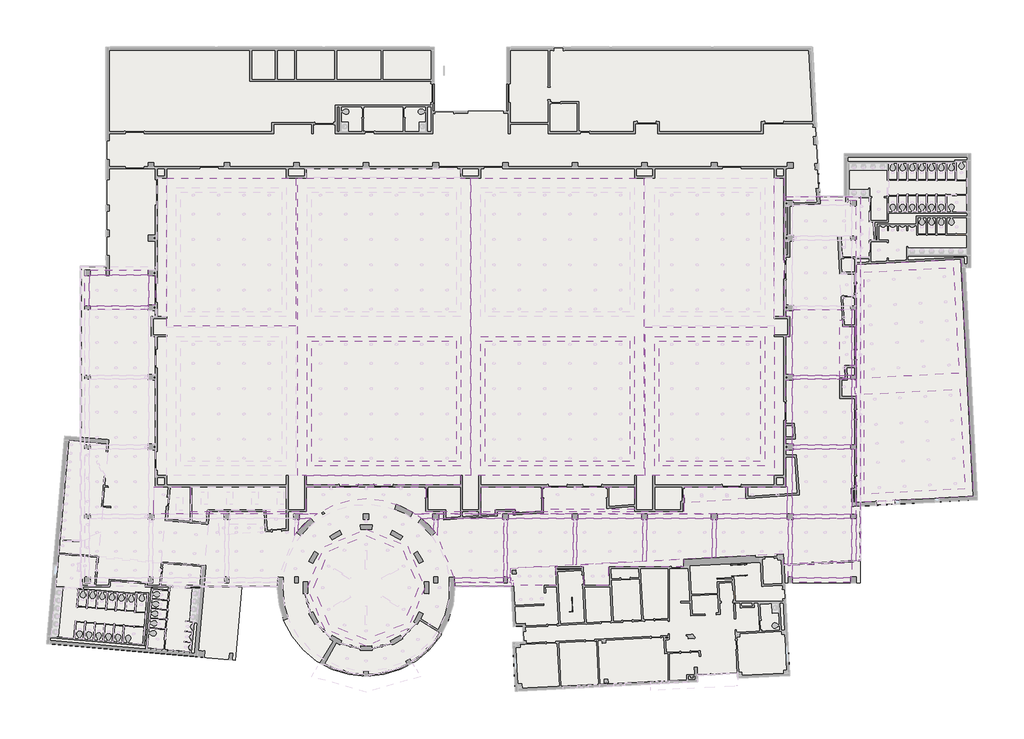
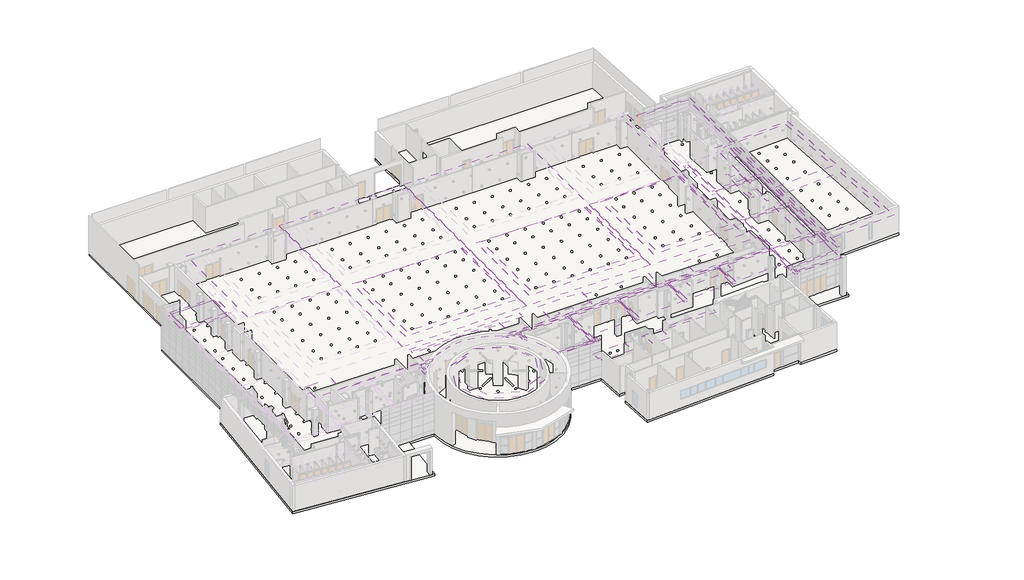
# One storey, part 23 of 30: 71 coverings, 1 slab.
"""IFC4 building model written with IfcOpenShell, lengths in millimetres."""

from ifc_helpers import new_model, si_unit, point, frame, frame_2d, origin, place, context, project, spatial, polyline, circle_curve, trimmed, segment, composite_curve, outline, extrude, faceted_brep, element, save

model = new_model("IFC4")

# Units and contexts
model_context = context("Model", 3, world=origin())
ifc_project = project(units=[si_unit("LENGTHUNIT", "METRE", prefix="MILLI")], contexts=[model_context])

# Site, building, storey
site = spatial("IfcSite", under=ifc_project)
building = spatial("IfcBuilding", under=site)
storey = spatial("IfcBuildingStorey", under=building, Name="1ST. FL.", Elevation=0.0)

# Coverings
placement = place(None, origin())
element("IfcCovering", 1, ObjectType="2' x 2' ACT System", at=placement, inside=storey, context=model_context, shape_type="SweptSolid", body=[
    extrude(outline(polyline([(-29897.3440345, -14000.959635), (-29897.3440345, -2418.559635), (-15978.1440345, -2418.559635), (-15978.1440345, -14000.959635), (-29897.3440345, -14000.959635)])), frame((0.0, 0.0, 6096.0), z_axis=(0.0, 0.0, 1.0), x_axis=(1.0, 0.0, 0.0)), (0.0, 0.0, 1.0), 50.8),
])
element("IfcCovering", 2, ObjectType="2' x 2' ACT System", at=placement, inside=storey, context=model_context, shape_type="SweptSolid", body=[
    extrude(outline(polyline([(13333.4559655, -14000.959635), (3579.8559655, -14000.959635), (3579.8559655, -2418.559635), (13333.4559655, -2418.559635), (13333.4559655, -14000.959635)])), frame((0.0, 0.0, 6096.0), z_axis=(0.0, 0.0, 1.0), x_axis=(1.0, 0.0, 0.0)), (0.0, 0.0, 1.0), 50.8),
])
element("IfcCovering", 3, ObjectType="2' x 2' ACT System", at=placement, inside=storey, context=model_context, shape_type="SweptSolid", body=[
    extrude(outline(polyline([(735.0559655, -14000.959635), (-13184.1440345, -14000.959635), (-13184.1440345, -2418.559635), (735.0559655, -2418.559635), (735.0559655, -14000.959635)])), frame((0.0, 0.0, 6096.0), z_axis=(0.0, 0.0, 1.0), x_axis=(1.0, 0.0, 0.0)), (0.0, 0.0, 1.0), 50.8),
])
element("IfcCovering", 4, ObjectType="2' x 2' ACT System", at=placement, inside=storey, context=model_context, shape_type="SweptSolid", body=[
    extrude(outline(polyline([(16476.7059655, -5717.384635), (16476.7059655, -5625.309635), (16384.6309655, -5625.309635), (16384.6309655, 534.190365), (16476.7059655, 534.190365), (16476.7059655, 626.265365), (22118.6809655, 626.265365), (22118.6809655, -5717.384635), (16476.7059655, -5717.384635)])), frame((0.0, 0.0, 5181.6), z_axis=(0.0, 0.0, 1.0), x_axis=(1.0, 0.0, 0.0)), (0.0, 0.0, 1.0), 50.8),
])
element("IfcCovering", 5, ObjectType="2' x 2' ACT System", at=placement, inside=storey, context=model_context, shape_type="SweptSolid", body=[
    extrude(outline(polyline([(16476.7059655, -6079.334635), (22118.6809655, -6079.334635), (22118.6809655, -12422.984635), (16476.7059655, -12422.984635), (16476.7059655, -12330.909635), (16384.6309655, -12330.909635), (16384.6309655, -6171.409635), (16476.7059655, -6171.409635), (16476.7059655, -6079.334635)])), frame((0.0, 0.0, 5181.6), z_axis=(0.0, 0.0, 1.0), x_axis=(1.0, 0.0, 0.0)), (0.0, 0.0, 1.0), 50.8),
])
element("IfcCovering", 6, ObjectType="2' x 2' ACT System", at=placement, inside=storey, context=model_context, shape_type="SweptSolid", body=[
    extrude(outline(polyline([(16476.7059655, -19128.584635), (16476.7059655, -19036.509635), (16384.6309655, -19036.509635), (16384.6309655, -12877.009635), (16476.7059655, -12877.009635), (16476.7059655, -12784.934635), (22118.6809655, -12784.934635), (22118.6809655, -19128.584635), (16476.7059655, -19128.584635)])), frame((0.0, 0.0, 5181.6), z_axis=(0.0, 0.0, 1.0), x_axis=(1.0, 0.0, 0.0)), (0.0, 0.0, 1.0), 50.8),
])
element("IfcCovering", 7, ObjectType="2' x 2' ACT System", at=placement, inside=storey, context=model_context, shape_type="SweptSolid", body=[
    extrude(outline(polyline([(16476.7059655, -19490.534635), (22118.6809655, -19490.534635), (22118.6809655, -23584.9151815), (16384.6309655, -23885.4240083), (16384.6309655, -19582.609635), (16476.7059655, -19582.609635), (16476.7059655, -19490.534635)])), frame((0.0, 0.0, 5181.6), z_axis=(0.0, 0.0, 1.0), x_axis=(1.0, 0.0, 0.0)), (0.0, 0.0, 1.0), 50.8),
])
element("IfcCovering", 8, ObjectType="2' x 2' ACT System", at=placement, inside=storey, context=model_context, shape_type="SweptSolid", body=[
    extrude(outline(polyline([(15930.6059655, -19490.534635), (15930.6059655, -19582.609635), (16022.6809655, -19582.609635), (16022.6809655, -23904.393004), (15588.5919456, -23927.1426455), (15535.7509474, -22918.8763358), (9069.4309655, -23257.7618061), (9069.4309655, -19582.609635), (9161.5059655, -19582.609635), (9161.5059655, -19490.534635), (15930.6059655, -19490.534635)])), frame((0.0, 0.0, 5181.6), z_axis=(0.0, 0.0, 1.0), x_axis=(1.0, 0.0, 0.0)), (0.0, 0.0, 1.0), 50.8),
])
element("IfcCovering", 9, ObjectType="2' x 2' ACT System", at=placement, inside=storey, context=model_context, shape_type="SweptSolid", body=[
    extrude(outline(polyline([(2455.9059655, -19490.534635), (8615.4059655, -19490.534635), (8615.4059655, -19582.609635), (8707.4809655, -19582.609635), (8707.4809655, -23276.7308019), (2363.8309655, -23609.1874109), (2363.8309655, -19582.609635), (2455.9059655, -19582.609635), (2455.9059655, -19490.534635)])), frame((0.0, 0.0, 5181.6), z_axis=(0.0, 0.0, 1.0), x_axis=(1.0, 0.0, 0.0)), (0.0, 0.0, 1.0), 50.8),
])
element("IfcCovering", 10, ObjectType="2' x 2' ACT System", at=placement, inside=storey, context=model_context, shape_type="SweptSolid", body=[
    extrude(outline(polyline([(1909.8059655, -19490.534635), (1909.8059655, -19582.609635), (2001.8809655, -19582.609635), (2001.8809655, -23628.1564066), (-4341.7690345, -23960.6130157), (-4341.7690345, -19582.609635), (-4249.6940345, -19582.609635), (-4249.6940345, -19490.534635), (1909.8059655, -19490.534635)])), frame((0.0, 0.0, 5181.6), z_axis=(0.0, 0.0, 1.0), x_axis=(1.0, 0.0, 0.0)), (0.0, 0.0, 1.0), 50.8),
])
element("IfcCovering", 11, ObjectType="2' x 2' ACT System", at=placement, inside=storey, context=model_context, shape_type="SweptSolid", body=[
    extrude(outline(polyline([(-10955.2940345, -19490.534635), (-4795.7940345, -19490.534635), (-4795.7940345, -19582.609635), (-4703.7190345, -19582.609635), (-4703.7190345, -23979.5820114), (-10767.9512721, -24297.394956), (-10719.3593201, -25224.584635), (-11047.3690345, -25224.584635), (-11047.3690345, -19582.609635), (-10955.2940345, -19582.609635), (-10955.2940345, -19490.534635)])), frame((0.0, 0.0, 5181.6), z_axis=(0.0, 0.0, 1.0), x_axis=(1.0, 0.0, 0.0)), (0.0, 0.0, 1.0), 50.8),
])
element("IfcCovering", 12, ObjectType="2' x 2' ACT System", at=placement, inside=storey, context=model_context, shape_type="SweptSolid", body=[
    extrude(outline(polyline([(-45638.9940345, 3979.065365), (-45638.9940345, 3886.990365), (-45546.9190345, 3886.990365), (-45546.9190345, 1080.290365), (-45638.9940345, 1080.290365), (-45638.9940345, 988.215365), (-51280.9690345, 988.215365), (-51280.9690345, 3886.990365), (-51188.8940345, 3886.990365), (-51188.8940345, 3979.065365), (-45638.9940345, 3979.065365)])), frame((0.0, 0.0, 5181.6), z_axis=(0.0, 0.0, 1.0), x_axis=(1.0, 0.0, 0.0)), (0.0, 0.0, 1.0), 50.8),
])
element("IfcCovering", 13, ObjectType="2' x 2' ACT System", at=placement, inside=storey, context=model_context, shape_type="SweptSolid", body=[
    extrude(outline(composite_curve([segment(polyline([(-31072.0940345, -19490.534635), (-29954.9292989, -19490.534635)]), True, "CONTINUOUS"), segment(trimmed(circle_curve(frame_2d((-24639.5440345, -26167.559635)), 8534.4), [point((-29954.9292989, -19490.534635))], [point((-31164.1690345, -20666.1732671))], True, "CARTESIAN"), True, "CONTINUOUS"), segment(polyline([(-31164.1690345, -20666.1732671), (-31164.1690345, -19582.609635), (-31072.0940345, -19582.609635), (-31072.0940345, -19490.534635)]), True, "CONTINUOUS")], self_intersect=False)), frame((0.0, 0.0, 5181.6), z_axis=(0.0, 0.0, 1.0), x_axis=(1.0, 0.0, 0.0)), (0.0, 0.0, 1.0), 50.8),
])
element("IfcCovering", 14, ObjectType="2' x 2' ACT System", at=placement, inside=storey, context=model_context, shape_type="SweptSolid", body=[
    extrude(outline(composite_curve([segment(polyline([(-18206.9940345, -19490.534635), (-18206.9940345, -19582.609635), (-18114.9190345, -19582.609635), (-18114.9190345, -20666.1732671)]), True, "CONTINUOUS"), segment(trimmed(circle_curve(frame_2d((-24639.5440345, -26167.559635)), 8534.4), [point((-18114.9190345, -20666.1732671))], [point((-19324.1587701, -19490.534635))], True, "CARTESIAN"), True, "CONTINUOUS"), segment(polyline([(-19324.1587701, -19490.534635), (-18206.9940345, -19490.534635)]), True, "CONTINUOUS")], self_intersect=False)), frame((0.0, 0.0, 5181.6), z_axis=(0.0, 0.0, 1.0), x_axis=(1.0, 0.0, 0.0)), (0.0, 0.0, 1.0), 50.8),
])
element("IfcCovering", 15, ObjectType="2' x 2' ACT System", at=placement, inside=storey, context=model_context, shape_type="SweptSolid", body=[
    extrude(outline(composite_curve([segment(polyline([(-17660.8940345, -19490.534635), (-11501.3940345, -19490.534635), (-11501.3940345, -19582.609635), (-11409.3190345, -19582.609635), (-11409.3190345, -25224.584635), (-16157.3991696, -25224.584635)]), True, "CONTINUOUS"), segment(trimmed(circle_curve(frame_2d((-24639.5440345, -26167.559635)), 8534.4), [point((-16157.3991696, -25224.584635))], [point((-17752.9690345, -21126.620424))], True, "CARTESIAN"), True, "CONTINUOUS"), segment(polyline([(-17752.9690345, -21126.620424), (-17752.9690345, -19582.609635), (-17660.8940345, -19582.609635), (-17660.8940345, -19490.534635)]), True, "CONTINUOUS")], self_intersect=False)), frame((0.0, 0.0, 5181.6), z_axis=(0.0, 0.0, 1.0), x_axis=(1.0, 0.0, 0.0)), (0.0, 0.0, 1.0), 50.8),
])
element("IfcCovering", 16, ObjectType="2' x 2' ACT System", at=placement, inside=storey, context=model_context, shape_type="SweptSolid", body=[
    extrude(outline(polyline([(31909.2771996, 4687.1559255), (32443.7073352, -5510.3785431), (23334.7059655, -5987.7610764), (23334.7059655, 4237.7816888), (31909.2771996, 4687.1559255)])), frame((0.0, 0.0, 2743.2), z_axis=(0.0, 0.0, 1.0), x_axis=(1.0, 0.0, 0.0)), (0.0, 0.0, 1.0), 50.8),
])
element("IfcCovering", 17, ObjectType="2' x 2' ACT System", at=placement, inside=storey, context=model_context, shape_type="SweptSolid", body=[
    extrude(outline(polyline([(32523.4673326, -7032.2899541), (33027.0803286, -16641.7983694), (23334.7059655, -17149.7541858), (23334.7059655, -7513.8525317), (32523.4673326, -7032.2899541)])), frame((0.0, 0.0, 2743.2), z_axis=(0.0, 0.0, 1.0), x_axis=(1.0, 0.0, 0.0)), (0.0, 0.0, 1.0), 50.8),
])
element("IfcCovering", 18, ObjectType="GWB on Mtl. Stud", at=placement, inside=storey, context=model_context, shape_type="SweptSolid", body=[
    extrude(outline(polyline([(15594.0559655, -56.359635), (14679.6559655, -56.359635), (14679.6559655, 13304.040365), (15594.0559655, 13304.040365), (15594.0559655, -56.359635)])), frame((0.0, 0.0, 4572.0), z_axis=(0.0, 0.0, 1.0), x_axis=(1.0, 0.0, 0.0)), (0.0, 0.0, 1.0), 50.8),
    extrude(outline(polyline([(15594.0559655, -1986.759635), (15594.0559655, -15347.159635), (14679.6559655, -15347.159635), (14679.6559655, -1986.759635), (15594.0559655, -1986.759635)])), frame((0.0, 0.0, 4572.0), z_axis=(0.0, 0.0, 1.0), x_axis=(1.0, 0.0, 0.0)), (0.0, 0.0, 1.0), 50.8),
])
element("IfcCovering", 19, ObjectType="GWB on Mtl. Stud", at=placement, inside=storey, context=model_context, shape_type="Brep", body=[
    faceted_brep([(3148.0559655, -16261.559635, 4622.8), (14679.6559655, -16261.559635, 4622.8), (14679.6559655, -15397.959635, 4622.8), (14679.6559655, -15347.159635, 4622.8), (3148.0559655, -15347.159635, 4622.8), (3148.0559655, -15397.959635, 4622.8), (3148.0559655, -16261.559635, 4572.0), (3148.0559655, -15347.159635, 4572.0), (14679.6559655, -15347.159635, 4572.0), (14679.6559655, -16261.559635, 4572.0)], [[[0, 1, 2, 3, 4, 5]], [[6, 7, 8, 9]], [[1, 0, 6, 9]], [[3, 2, 1, 9, 8]], [[4, 3, 8, 7]], [[0, 5, 4, 7, 6]]]),
    faceted_brep([(-30379.9440345, -16261.559635, 4622.8), (-15546.3440345, -16261.559635, 4622.8), (-15546.3440345, -15397.959635, 4622.8), (-15546.3440345, -15347.159635, 4622.8), (-30379.9440345, -15347.159635, 4622.8), (-30379.9440345, -15397.959635, 4622.8), (-30379.9440345, -16261.559635, 4572.0), (-30379.9440345, -15347.159635, 4572.0), (-15546.3440345, -15347.159635, 4572.0), (-15546.3440345, -16261.559635, 4572.0)], [[[0, 1, 2, 3, 4, 5]], [[6, 7, 8, 9]], [[1, 0, 6, 9]], [[3, 2, 1, 9, 8]], [[4, 3, 8, 7]], [[0, 5, 4, 7, 6]]]),
    faceted_brep([(-43841.9440345, -16261.559635, 4622.8), (-32310.3440345, -16261.559635, 4622.8), (-32310.3440345, -15397.959635, 4622.8), (-32310.3440345, -15347.159635, 4622.8), (-43841.9440345, -15347.159635, 4622.8), (-43841.9440345, -15397.959635, 4622.8), (-43841.9440345, -16261.559635, 4572.0), (-43841.9440345, -15347.159635, 4572.0), (-32310.3440345, -15347.159635, 4572.0), (-32310.3440345, -16261.559635, 4572.0)], [[[0, 1, 2, 3, 4, 5]], [[6, 7, 8, 9]], [[1, 0, 6, 9]], [[3, 2, 1, 9, 8]], [[4, 3, 8, 7]], [[0, 5, 4, 7, 6]]]),
    faceted_brep([(1217.6559655, -16261.559635, 4622.8), (1217.6559655, -15397.959635, 4622.8), (1217.6559655, -15347.159635, 4622.8), (-13615.9440345, -15347.159635, 4622.8), (-13615.9440345, -15397.959635, 4622.8), (-13615.9440345, -16261.559635, 4622.8), (1217.6559655, -16261.559635, 4572.0), (-13615.9440345, -16261.559635, 4572.0), (-13615.9440345, -15347.159635, 4572.0), (1217.6559655, -15347.159635, 4572.0)], [[[0, 1, 2, 3, 4, 5]], [[6, 7, 8, 9]], [[2, 1, 0, 6, 9]], [[3, 2, 9, 8]], [[5, 4, 3, 8, 7]], [[0, 5, 7, 6]]]),
])
element("IfcCovering", 20, ObjectType="GWB on Mtl. Stud", at=placement, inside=storey, context=model_context, shape_type="SweptSolid", body=[
    extrude(outline(polyline([(-43841.9440345, 13304.040365), (-31395.9440345, 13304.040365), (-31395.9440345, -970.759635), (-43841.9440345, -970.759635), (-43841.9440345, 13304.040365)]), holes=[polyline([(-32310.3440345, -56.359635), (-32310.3440345, 12389.640365), (-42927.5440345, 12389.640365), (-42927.5440345, -56.359635), (-32310.3440345, -56.359635)])]), frame((0.0, 0.0, 5181.6), z_axis=(0.0, 0.0, 1.0), x_axis=(1.0, 0.0, 0.0)), (0.0, 0.0, 1.0), 50.8),
])
element("IfcCovering", 21, ObjectType="GWB on Mtl. Stud", at=placement, inside=storey, context=model_context, shape_type="Brep", body=[
    faceted_brep([(-31243.5440345, -15347.159635, 5232.4), (-30379.9440345, -15347.159635, 5232.4), (-15546.3440345, -15347.159635, 5232.4), (-14631.9440345, -15347.159635, 5232.4), (-14631.9440345, 13304.040365, 5232.4), (-15546.3440345, 13304.040365, 5232.4), (-30379.9440345, 13304.040365, 5232.4), (-31243.5440345, 13304.040365, 5232.4), (-15546.3440345, -14432.759635, 5232.4), (-30329.1440345, -14432.759635, 5232.4), (-30329.1440345, -1986.759635, 5232.4), (-15546.3440345, -1986.759635, 5232.4), (-15495.5440345, 12440.440365, 5232.4), (-15495.5440345, -107.159635, 5232.4), (-30379.9440345, -107.159635, 5232.4), (-30379.9440345, 12440.440365, 5232.4), (-14631.9440345, -15347.159635, 5181.6), (-31243.5440345, -15347.159635, 5181.6), (-31243.5440345, 13304.040365, 5181.6), (-14631.9440345, 13304.040365, 5181.6), (-30329.1440345, -14432.759635, 5181.6), (-15546.3440345, -14432.759635, 5181.6), (-15546.3440345, -1986.759635, 5181.6), (-30329.1440345, -1986.759635, 5181.6), (-15495.5440345, -107.159635, 5181.6), (-15495.5440345, 12440.440365, 5181.6), (-30379.9440345, 12440.440365, 5181.6), (-30379.9440345, -107.159635, 5181.6)], [[[0, 1, 2, 3, 4, 5, 6, 7], [8, 9, 10, 11], [12, 13, 14, 15]], [[16, 17, 18, 19], [20, 21, 22, 23], [24, 25, 26, 27]], [[9, 8, 21, 20]], [[10, 9, 20, 23]], [[11, 10, 23, 22]], [[3, 2, 1, 0, 17, 16]], [[0, 7, 18, 17]], [[8, 11, 22, 21]], [[4, 3, 16, 19]], [[7, 6, 5, 4, 19, 18]], [[24, 13, 12, 25]], [[25, 12, 15, 26]], [[26, 15, 14, 27]], [[13, 24, 27, 14]]]),
])
element("IfcCovering", 22, ObjectType="GWB on Mtl. Stud", at=placement, inside=storey, context=model_context, shape_type="SweptSolid", body=[
    extrude(outline(polyline([(-15546.3440345, -14432.759635), (-30329.1440345, -14432.759635), (-30329.1440345, -1986.759635), (-15546.3440345, -1986.759635), (-15546.3440345, -14432.759635)]), holes=[polyline([(-29948.1440345, -14051.759635), (-15927.3440345, -14051.759635), (-15927.3440345, -2367.759635), (-29948.1440345, -2367.759635), (-29948.1440345, -14051.759635)])]), frame((0.0, 0.0, 5791.2), z_axis=(0.0, 0.0, 1.0), x_axis=(1.0, 0.0, 0.0)), (0.0, 0.0, 1.0), 50.8),
])
element("IfcCovering", 23, ObjectType="GWB on Mtl. Stud", at=placement, inside=storey, context=model_context, shape_type="SweptSolid", body=[
    extrude(outline(polyline([(14679.6559655, -15347.159635), (2233.6559655, -15347.159635), (2233.6559655, -1072.359635), (14679.6559655, -1072.359635), (14679.6559655, -15347.159635)]), holes=[polyline([(3148.0559655, -1986.759635), (3148.0559655, -14432.759635), (13765.2559655, -14432.759635), (13765.2559655, -1986.759635), (3148.0559655, -1986.759635)])]), frame((0.0, 0.0, 5181.6), z_axis=(0.0, 0.0, 1.0), x_axis=(1.0, 0.0, 0.0)), (0.0, 0.0, 1.0), 50.8),
])
element("IfcCovering", 24, ObjectType="GWB on Mtl. Stud", at=placement, inside=storey, context=model_context, shape_type="SweptSolid", body=[
    extrude(outline(polyline([(2081.2559655, -15347.159635), (-14530.3440345, -15347.159635), (-14530.3440345, 13304.040365), (2081.2559655, 13304.040365), (2081.2559655, -15347.159635)]), holes=[polyline([(-13615.9440345, -1986.759635), (-13615.9440345, -14432.759635), (1166.8559655, -14432.759635), (1166.8559655, -1986.759635), (-13615.9440345, -1986.759635)]), polyline([(-13615.9440345, -56.359635), (1166.8559655, -56.359635), (1166.8559655, 12389.640365), (-13615.9440345, 12389.640365), (-13615.9440345, -56.359635)])]), frame((0.0, 0.0, 5181.6), z_axis=(0.0, 0.0, 1.0), x_axis=(1.0, 0.0, 0.0)), (0.0, 0.0, 1.0), 50.8),
])
element("IfcCovering", 25, ObjectType="GWB on Mtl. Stud", at=placement, inside=storey, context=model_context, shape_type="SweptSolid", body=[
    extrude(outline(polyline([(3148.0559655, -1986.759635), (13765.2559655, -1986.759635), (13765.2559655, -14432.759635), (3148.0559655, -14432.759635), (3148.0559655, -1986.759635)]), holes=[polyline([(3579.8559655, -2418.559635), (3579.8559655, -14000.959635), (13333.4559655, -14000.959635), (13333.4559655, -2418.559635), (3579.8559655, -2418.559635)])]), frame((0.0, 0.0, 5791.2), z_axis=(0.0, 0.0, 1.0), x_axis=(1.0, 0.0, 0.0)), (0.0, 0.0, 1.0), 50.8),
])
element("IfcCovering", 26, ObjectType="GWB on Mtl. Stud", at=placement, inside=storey, context=model_context, shape_type="SweptSolid", body=[
    extrude(outline(polyline([(-13615.9440345, -1986.759635), (1166.8559655, -1986.759635), (1166.8559655, -14432.759635), (-13615.9440345, -14432.759635), (-13615.9440345, -1986.759635)]), holes=[polyline([(-13184.1440345, -2418.559635), (-13184.1440345, -14000.959635), (735.0559655, -14000.959635), (735.0559655, -2418.559635), (-13184.1440345, -2418.559635)])]), frame((0.0, 0.0, 5791.2), z_axis=(0.0, 0.0, 1.0), x_axis=(1.0, 0.0, 0.0)), (0.0, 0.0, 1.0), 50.8),
])
element("IfcCovering", 27, ObjectType="GWB on Mtl. Stud", at=placement, inside=storey, context=model_context, shape_type="SweptSolid", body=[
    extrude(outline(polyline([(22026.6059655, -6079.334635), (16476.7059655, -6079.334635), (16476.7059655, -5717.384635), (22026.6059655, -5717.384635), (22026.6059655, -6079.334635)])), frame((0.0, 0.0, 4895.85), z_axis=(0.0, 0.0, 1.0), x_axis=(1.0, 0.0, 0.0)), (0.0, 0.0, 1.0), 50.8),
])
element("IfcCovering", 28, ObjectType="GWB on Mtl. Stud", at=placement, inside=storey, context=model_context, shape_type="SweptSolid", body=[
    extrude(outline(polyline([(22026.6059655, -12784.934635), (16476.7059655, -12784.934635), (16476.7059655, -12422.984635), (22026.6059655, -12422.984635), (22026.6059655, -12784.934635)])), frame((0.0, 0.0, 4895.85), z_axis=(0.0, 0.0, 1.0), x_axis=(1.0, 0.0, 0.0)), (0.0, 0.0, 1.0), 50.8),
])
element("IfcCovering", 29, ObjectType="GWB on Mtl. Stud", at=placement, inside=storey, context=model_context, shape_type="SweptSolid", body=[
    extrude(outline(polyline([(22026.6059655, -19490.534635), (16476.7059655, -19490.534635), (16476.7059655, -19128.584635), (22026.6059655, -19128.584635), (22026.6059655, -19490.534635)])), frame((0.0, 0.0, 4895.85), z_axis=(0.0, 0.0, 1.0), x_axis=(1.0, 0.0, 0.0)), (0.0, 0.0, 1.0), 50.8),
])
element("IfcCovering", 30, ObjectType="GWB on Mtl. Stud", at=placement, inside=storey, context=model_context, shape_type="SweptSolid", body=[
    extrude(outline(polyline([(22572.7059655, -5717.384635), (22118.6809655, -5717.384635), (22118.6809655, 626.265365), (22572.7059655, 626.265365), (22572.7059655, -5717.384635)])), frame((0.0, 0.0, 5118.1), z_axis=(0.0, 0.0, 1.0), x_axis=(1.0, 0.0, 0.0)), (0.0, 0.0, 1.0), 50.8),
])
element("IfcCovering", 31, ObjectType="GWB on Mtl. Stud", at=placement, inside=storey, context=model_context, shape_type="SweptSolid", body=[
    extrude(outline(polyline([(16384.6309655, -5625.309635), (15771.8559655, -5625.309635), (15771.8559655, -1986.759635), (16159.2059655, -1986.759635), (16159.2059655, -56.359635), (15771.8559655, -56.359635), (15771.8559655, 534.190365), (16384.6309655, 534.190365), (16384.6309655, -5625.309635)])), frame((0.0, 0.0, 4895.85), z_axis=(0.0, 0.0, 1.0), x_axis=(1.0, 0.0, 0.0)), (0.0, 0.0, 1.0), 50.8),
])
element("IfcCovering", 32, ObjectType="GWB on Mtl. Stud", at=placement, inside=storey, context=model_context, shape_type="SweptSolid", body=[
    extrude(outline(polyline([(22572.7059655, -12422.984635), (22118.6809655, -12422.984635), (22118.6809655, -6079.334635), (22572.7059655, -6079.334635), (22572.7059655, -12422.984635)])), frame((0.0, 0.0, 5118.1), z_axis=(0.0, 0.0, 1.0), x_axis=(1.0, 0.0, 0.0)), (0.0, 0.0, 1.0), 50.8),
])
element("IfcCovering", 33, ObjectType="GWB on Mtl. Stud", at=placement, inside=storey, context=model_context, shape_type="SweptSolid", body=[
    extrude(outline(polyline([(16384.6309655, -12330.909635), (15771.8559655, -12330.909635), (15771.8559655, -6171.409635), (16384.6309655, -6171.409635), (16384.6309655, -12330.909635)])), frame((0.0, 0.0, 4895.85), z_axis=(0.0, 0.0, 1.0), x_axis=(1.0, 0.0, 0.0)), (0.0, 0.0, 1.0), 50.8),
])
element("IfcCovering", 34, ObjectType="GWB on Mtl. Stud", at=placement, inside=storey, context=model_context, shape_type="SweptSolid", body=[
    extrude(outline(polyline([(22572.7059655, -19128.584635), (22118.6809655, -19128.584635), (22118.6809655, -12784.934635), (22572.7059655, -12784.934635), (22572.7059655, -19128.584635)])), frame((0.0, 0.0, 5118.1), z_axis=(0.0, 0.0, 1.0), x_axis=(1.0, 0.0, 0.0)), (0.0, 0.0, 1.0), 50.8),
])
element("IfcCovering", 35, ObjectType="GWB on Mtl. Stud", at=placement, inside=storey, context=model_context, shape_type="SweptSolid", body=[
    extrude(outline(polyline([(16384.6309655, -19036.509635), (15930.6059655, -19036.509635), (15930.6059655, -16439.359635), (15771.8559655, -16439.359635), (15771.8559655, -12877.009635), (16384.6309655, -12877.009635), (16384.6309655, -19036.509635)])), frame((0.0, 0.0, 4895.85), z_axis=(0.0, 0.0, 1.0), x_axis=(1.0, 0.0, 0.0)), (0.0, 0.0, 1.0), 50.8),
])
element("IfcCovering", 36, ObjectType="GWB on Mtl. Stud", at=placement, inside=storey, context=model_context, shape_type="SweptSolid", body=[
    extrude(outline(polyline([(22572.7059655, -23561.1207395), (22118.6809655, -23584.9151815), (22118.6809655, -19490.534635), (22572.7059655, -19490.534635), (22572.7059655, -23561.1207395)])), frame((0.0, 0.0, 5118.1), z_axis=(0.0, 0.0, 1.0), x_axis=(1.0, 0.0, 0.0)), (0.0, 0.0, 1.0), 50.8),
])
element("IfcCovering", 37, ObjectType="GWB on Mtl. Stud", at=placement, inside=storey, context=model_context, shape_type="SweptSolid", body=[
    extrude(outline(polyline([(16384.6309655, -23885.4240083), (16022.6809655, -23904.393004), (16022.6809655, -19582.609635), (16384.6309655, -19582.609635), (16384.6309655, -23885.4240083)])), frame((0.0, 0.0, 4895.85), z_axis=(0.0, 0.0, 1.0), x_axis=(1.0, 0.0, 0.0)), (0.0, 0.0, 1.0), 50.8),
])
element("IfcCovering", 38, ObjectType="GWB on Mtl. Stud", at=placement, inside=storey, context=model_context, shape_type="SweptSolid", body=[
    extrude(outline(polyline([(15930.6059655, -19490.534635), (9161.5059655, -19490.534635), (9161.5059655, -19036.509635), (15930.6059655, -19036.509635), (15930.6059655, -19490.534635)])), frame((0.0, 0.0, 4895.85), z_axis=(0.0, 0.0, 1.0), x_axis=(1.0, 0.0, 0.0)), (0.0, 0.0, 1.0), 50.8),
])
element("IfcCovering", 39, ObjectType="GWB on Mtl. Stud", at=placement, inside=storey, context=model_context, shape_type="SweptSolid", body=[
    extrude(outline(polyline([(8615.4059655, -19490.534635), (2455.9059655, -19490.534635), (2455.9059655, -19036.509635), (8615.4059655, -19036.509635), (8615.4059655, -19490.534635)])), frame((0.0, 0.0, 4895.85), z_axis=(0.0, 0.0, 1.0), x_axis=(1.0, 0.0, 0.0)), (0.0, 0.0, 1.0), 50.8),
])
element("IfcCovering", 40, ObjectType="GWB on Mtl. Stud", at=placement, inside=storey, context=model_context, shape_type="SweptSolid", body=[
    extrude(outline(polyline([(1909.8059655, -19490.534635), (-4249.6940345, -19490.534635), (-4249.6940345, -19036.509635), (1909.8059655, -19036.509635), (1909.8059655, -19490.534635)])), frame((0.0, 0.0, 4895.85), z_axis=(0.0, 0.0, 1.0), x_axis=(1.0, 0.0, 0.0)), (0.0, 0.0, 1.0), 50.8),
])
element("IfcCovering", 41, ObjectType="GWB on Mtl. Stud", at=placement, inside=storey, context=model_context, shape_type="SweptSolid", body=[
    extrude(outline(polyline([(-4795.7940345, -19490.534635), (-10955.2940345, -19490.534635), (-10955.2940345, -19036.509635), (-4795.7940345, -19036.509635), (-4795.7940345, -19490.534635)])), frame((0.0, 0.0, 4895.85), z_axis=(0.0, 0.0, 1.0), x_axis=(1.0, 0.0, 0.0)), (0.0, 0.0, 1.0), 50.8),
])
element("IfcCovering", 42, ObjectType="GWB on Mtl. Stud", at=placement, inside=storey, context=model_context, shape_type="SweptSolid", body=[
    extrude(outline(polyline([(-11501.3940345, -19490.534635), (-17660.8940345, -19490.534635), (-17660.8940345, -19036.509635), (-11501.3940345, -19036.509635), (-11501.3940345, -19490.534635)])), frame((0.0, 0.0, 4895.85), z_axis=(0.0, 0.0, 1.0), x_axis=(1.0, 0.0, 0.0)), (0.0, 0.0, 1.0), 50.8),
])
element("IfcCovering", 43, ObjectType="GWB on Mtl. Stud", at=placement, inside=storey, context=model_context, shape_type="SweptSolid", body=[
    extrude(outline(composite_curve([segment(polyline([(-18206.9940345, -19490.534635), (-19324.1587701, -19490.534635)]), True, "CONTINUOUS"), segment(trimmed(circle_curve(frame_2d((-24639.5440345, -26167.559635)), 8534.4), [point((-19324.1587701, -19490.534635))], [point((-19950.8225395, -19036.509635))], True, "CARTESIAN"), True, "CONTINUOUS"), segment(polyline([(-19950.8225395, -19036.509635), (-18206.9940345, -19036.509635), (-18206.9940345, -19490.534635)]), True, "CONTINUOUS")], self_intersect=False)), frame((0.0, 0.0, 4895.85), z_axis=(0.0, 0.0, 1.0), x_axis=(1.0, 0.0, 0.0)), (0.0, 0.0, 1.0), 50.8),
])
element("IfcCovering", 44, ObjectType="GWB on Mtl. Stud", at=placement, inside=storey, context=model_context, shape_type="SweptSolid", body=[
    extrude(outline(polyline([(-45546.9190345, 1080.290365), (-45546.9190345, 3886.990365), (-44934.1440345, 3886.990365), (-44934.1440345, 1080.290365), (-45546.9190345, 1080.290365)])), frame((0.0, 0.0, 4895.85), z_axis=(0.0, 0.0, 1.0), x_axis=(1.0, 0.0, 0.0)), (0.0, 0.0, 1.0), 50.8),
])
element("IfcCovering", 45, ObjectType="GWB on Mtl. Stud", at=placement, inside=storey, context=model_context, shape_type="SweptSolid", body=[
    extrude(outline(polyline([(9069.4309655, -23257.7618061), (8707.4809655, -23276.7308019), (8707.4809655, -19582.609635), (9069.4309655, -19582.609635), (9069.4309655, -23257.7618061)])), frame((0.0, 0.0, 4895.85), z_axis=(0.0, 0.0, 1.0), x_axis=(1.0, 0.0, 0.0)), (0.0, 0.0, 1.0), 50.8),
])
element("IfcCovering", 46, ObjectType="GWB on Mtl. Stud", at=placement, inside=storey, context=model_context, shape_type="SweptSolid", body=[
    extrude(outline(polyline([(2363.8309655, -23609.1874109), (2001.8809655, -23628.1564066), (2001.8809655, -19582.609635), (2363.8309655, -19582.609635), (2363.8309655, -23609.1874109)])), frame((0.0, 0.0, 4895.85), z_axis=(0.0, 0.0, 1.0), x_axis=(1.0, 0.0, 0.0)), (0.0, 0.0, 1.0), 50.8),
])
element("IfcCovering", 47, ObjectType="GWB on Mtl. Stud", at=placement, inside=storey, context=model_context, shape_type="SweptSolid", body=[
    extrude(outline(polyline([(-4341.7690345, -23960.6130157), (-4703.7190345, -23979.5820114), (-4703.7190345, -19582.609635), (-4341.7690345, -19582.609635), (-4341.7690345, -23960.6130157)])), frame((0.0, 0.0, 4895.85), z_axis=(0.0, 0.0, 1.0), x_axis=(1.0, 0.0, 0.0)), (0.0, 0.0, 1.0), 50.8),
])
element("IfcCovering", 48, ObjectType="GWB on Mtl. Stud", at=placement, inside=storey, context=model_context, shape_type="SweptSolid", body=[
    extrude(outline(polyline([(-11047.3690345, -25132.509635), (-11409.3190345, -25132.509635), (-11409.3190345, -19582.609635), (-11047.3690345, -19582.609635), (-11047.3690345, -25132.509635)])), frame((0.0, 0.0, 4895.85), z_axis=(0.0, 0.0, 1.0), x_axis=(1.0, 0.0, 0.0)), (0.0, 0.0, 1.0), 50.8),
])
element("IfcCovering", 49, ObjectType="GWB on Mtl. Stud", at=placement, inside=storey, context=model_context, shape_type="SweptSolid", body=[
    extrude(outline(polyline([(-45638.9940345, 626.265365), (-51188.8940345, 626.265365), (-51188.8940345, 988.215365), (-45638.9940345, 988.215365), (-45638.9940345, 626.265365)])), frame((0.0, 0.0, 4895.85), z_axis=(0.0, 0.0, 1.0), x_axis=(1.0, 0.0, 0.0)), (0.0, 0.0, 1.0), 50.8),
])
element("IfcCovering", 50, ObjectType="GWB on Mtl. Stud", at=placement, inside=storey, context=model_context, shape_type="SweptSolid", body=[
    extrude(outline(polyline([(-45638.9940345, 3979.065365), (-51188.8940345, 3979.065365), (-51188.8940345, 4433.090365), (-45638.9940345, 4433.090365), (-45638.9940345, 3979.065365)])), frame((0.0, 0.0, 5118.1), z_axis=(0.0, 0.0, 1.0), x_axis=(1.0, 0.0, 0.0)), (0.0, 0.0, 1.0), 50.8),
])
element("IfcCovering", 51, ObjectType="GWB on Mtl. Stud", at=placement, inside=storey, context=model_context, shape_type="SweptSolid", body=[
    extrude(outline(composite_curve([segment(polyline([(-31526.1190345, -19582.609635), (-31164.1690345, -19582.609635), (-31164.1690345, -20666.1732671)]), True, "CONTINUOUS"), segment(trimmed(circle_curve(frame_2d((-24639.5440345, -26167.559635)), 8534.4), [point((-31164.1690345, -20666.1732671))], [point((-31526.1190345, -21126.620424))], True, "CARTESIAN"), True, "CONTINUOUS"), segment(polyline([(-31526.1190345, -21126.620424), (-31526.1190345, -19582.609635)]), True, "CONTINUOUS")], self_intersect=False)), frame((0.0, 0.0, 4895.85), z_axis=(0.0, 0.0, 1.0), x_axis=(1.0, 0.0, 0.0)), (0.0, 0.0, 1.0), 50.8),
])
element("IfcCovering", 52, ObjectType="GWB on Mtl. Stud", at=placement, inside=storey, context=model_context, shape_type="SweptSolid", body=[
    extrude(outline(composite_curve([segment(polyline([(-18114.9190345, -19582.609635), (-17752.9690345, -19582.609635), (-17752.9690345, -21126.620424)]), True, "CONTINUOUS"), segment(trimmed(circle_curve(frame_2d((-24639.5440345, -26167.559635)), 8534.4), [point((-17752.9690345, -21126.620424))], [point((-18114.9190345, -20666.1732671))], True, "CARTESIAN"), True, "CONTINUOUS"), segment(polyline([(-18114.9190345, -20666.1732671), (-18114.9190345, -19582.609635)]), True, "CONTINUOUS")], self_intersect=False)), frame((0.0, 0.0, 4895.85), z_axis=(0.0, 0.0, 1.0), x_axis=(1.0, 0.0, 0.0)), (0.0, 0.0, 1.0), 50.8),
])
element("IfcCovering", 53, ObjectType="GWB on Mtl. Stud", at=placement, inside=storey, context=model_context, shape_type="SweptSolid", body=[
    extrude(outline(polyline([(-51280.9690345, 988.215365), (-51734.9940345, 988.215365), (-51734.9940345, 3886.990365), (-51280.9690345, 3886.990365), (-51280.9690345, 988.215365)])), frame((0.0, 0.0, 5118.1), z_axis=(0.0, 0.0, 1.0), x_axis=(1.0, 0.0, 0.0)), (0.0, 0.0, 1.0), 50.8),
])
element("IfcCovering", 54, ObjectType="GWB on Mtl. Stud", at=placement, inside=storey, context=model_context, shape_type="SweptSolid", body=[
    extrude(outline(composite_curve([segment(polyline([(-11409.3190345, -25224.584635), (-11409.3190345, -25678.609635), (-16119.161927, -25678.609635)]), True, "CONTINUOUS"), segment(trimmed(circle_curve(frame_2d((-24639.5440345, -26167.559635)), 8534.4), [point((-16119.161927, -25678.609635))], [point((-16157.3991696, -25224.584635))], True, "CARTESIAN"), True, "CONTINUOUS"), segment(polyline([(-16157.3991696, -25224.584635), (-11409.3190345, -25224.584635)]), True, "CONTINUOUS")], self_intersect=False)), frame((0.0, 0.0, 5118.1), z_axis=(0.0, 0.0, 1.0), x_axis=(1.0, 0.0, 0.0)), (0.0, 0.0, 1.0), 50.8),
])
element("IfcCovering", 55, ObjectType="GWB on Mtl. Stud", at=placement, inside=storey, context=model_context, shape_type="SweptSolid", body=[
    extrude(outline(composite_curve([segment(polyline([(-31072.0940345, -19490.534635), (-31072.0940345, -19036.509635), (-29328.2655295, -19036.509635)]), True, "CONTINUOUS"), segment(trimmed(circle_curve(frame_2d((-24639.5440345, -26167.559635)), 8534.4), [point((-29328.2655295, -19036.509635))], [point((-29954.9292989, -19490.534635))], True, "CARTESIAN"), True, "CONTINUOUS"), segment(polyline([(-29954.9292989, -19490.534635), (-31072.0940345, -19490.534635)]), True, "CONTINUOUS")], self_intersect=False)), frame((0.0, 0.0, 4895.85), z_axis=(0.0, 0.0, 1.0), x_axis=(1.0, 0.0, 0.0)), (0.0, 0.0, 1.0), 50.8),
])
element("IfcCovering", 56, ObjectType="GWB on Mtl. Stud", at=placement, inside=storey, context=model_context, shape_type="SweptSolid", body=[
    extrude(outline(composite_curve([segment(polyline([(-10676.9286718, -26034.209635), (-16106.185895, -26034.209635)]), True, "CONTINUOUS"), segment(trimmed(circle_curve(frame_2d((-24639.5440345, -26167.559635)), 8534.4), [point((-16106.185895, -26034.209635))], [point((-16119.161927, -25678.609635))], True, "CARTESIAN"), True, "CONTINUOUS"), segment(polyline([(-16119.161927, -25678.609635), (-10695.5648781, -25678.609635), (-10676.9286718, -26034.209635)]), True, "CONTINUOUS")], self_intersect=False)), frame((0.0, 0.0, 5505.45), z_axis=(0.0, 0.0, 1.0), x_axis=(1.0, 0.0, 0.0)), (0.0, 0.0, 1.0), 50.8),
])
element("IfcCovering", 57, ObjectType="GWB on Mtl. Stud", at=placement, inside=storey, context=model_context, shape_type="SweptSolid", body=[
    extrude(outline(polyline([(-11047.3690345, -25224.584635), (-10719.3593201, -25224.584635), (-10695.5648781, -25678.609635), (-11047.3690345, -25678.609635), (-11047.3690345, -25224.584635)])), frame((0.0, 0.0, 5118.1), z_axis=(0.0, 0.0, 1.0), x_axis=(1.0, 0.0, 0.0)), (0.0, 0.0, 1.0), 50.8),
])
element("IfcCovering", 58, ObjectType="GWB on Mtl. Stud", at=placement, inside=storey, context=model_context, shape_type="SweptSolid", body=[
    extrude(outline(polyline([(22928.3059655, -23542.4845332), (22572.7059655, -23561.1207395), (22572.7059655, 11138.690365), (15771.8559655, 11138.690365), (15771.8559655, 11494.290365), (22928.3059655, 11494.290365), (22928.3059655, -23542.4845332)])), frame((0.0, 0.0, 5505.45), z_axis=(0.0, 0.0, 1.0), x_axis=(1.0, 0.0, 0.0)), (0.0, 0.0, 1.0), 50.8),
])
element("IfcCovering", 59, ObjectType="GWB on Mtl. Stud", at=placement, inside=storey, context=model_context, shape_type="SweptSolid", body=[
    extrude(outline(polyline([(16384.6309655, -25132.509635), (16022.6809655, -25132.509635), (16022.6809655, -24037.9260063), (16384.6309655, -24018.9570106), (16384.6309655, -25132.509635)])), frame((0.0, 0.0, 4895.85), z_axis=(0.0, 0.0, 1.0), x_axis=(1.0, 0.0, 0.0)), (0.0, 0.0, 1.0), 50.8),
])
element("IfcCovering", 60, ObjectType="GWB on Mtl. Stud", at=placement, inside=storey, context=model_context, shape_type="SweptSolid", body=[
    extrude(outline(polyline([(22572.7059655, -25132.509635), (22118.6809655, -25132.509635), (22118.6809655, -23718.4481838), (22572.7059655, -23694.6537418), (22572.7059655, -25132.509635)])), frame((0.0, 0.0, 5505.45), z_axis=(0.0, 0.0, 1.0), x_axis=(1.0, 0.0, 0.0)), (0.0, 0.0, 1.0), 50.8),
    extrude(outline(polyline([(22026.6059655, -25678.609635), (16384.6309655, -25678.609635), (16384.6309655, -25224.584635), (22026.6059655, -25224.584635), (22026.6059655, -25678.609635)])), frame((0.0, 0.0, 5505.45), z_axis=(0.0, 0.0, 1.0), x_axis=(1.0, 0.0, 0.0)), (0.0, 0.0, 1.0), 50.8),
    extrude(outline(polyline([(15680.382441, -25678.609635), (15656.587999, -25224.584635), (16022.6809655, -25224.584635), (16022.6809655, -25678.609635), (15680.382441, -25678.609635)])), frame((0.0, 0.0, 5505.45), z_axis=(0.0, 0.0, 1.0), x_axis=(1.0, 0.0, 0.0)), (0.0, 0.0, 1.0), 50.8),
])
element("IfcCovering", 61, ObjectType="GWB on Mtl. Stud", at=placement, inside=storey, context=model_context, shape_type="SweptSolid", body=[
    extrude(outline(polyline([(22026.6059655, -25224.584635), (16384.6309655, -25224.584635), (16384.6309655, -24018.9570106), (22118.6809655, -23718.4481838), (22118.6809655, -25132.509635), (22026.6059655, -25132.509635), (22026.6059655, -25224.584635)])), frame((0.0, 0.0, 5181.6), z_axis=(0.0, 0.0, 1.0), x_axis=(1.0, 0.0, 0.0)), (0.0, 0.0, 1.0), 50.8),
    extrude(outline(polyline([(16022.6809655, -24037.9260063), (16022.6809655, -25224.584635), (15656.587999, -25224.584635), (15595.5709454, -24060.309894), (16022.6809655, -24037.9260063)])), frame((0.0, 0.0, 5181.6), z_axis=(0.0, 0.0, 1.0), x_axis=(1.0, 0.0, 0.0)), (0.0, 0.0, 1.0), 50.8),
])
element("IfcCovering", 62, ObjectType="GWB on Mtl. Stud", at=placement, inside=storey, context=model_context, shape_type="SweptSolid", body=[
    extrude(outline(composite_curve([segment(polyline([(15930.6059655, -19036.509635), (-19950.8225395, -19036.509635)]), True, "CONTINUOUS"), segment(trimmed(circle_curve(frame_2d((-24639.5440345, -26167.559635)), 8534.4), [point((-19950.8225395, -19036.509635))], [point((-29328.2655295, -19036.509635))], True, "CARTESIAN"), True, "CONTINUOUS"), segment(polyline([(-29328.2655295, -19036.509635), (-45092.8940345, -19036.509635), (-45092.8940345, -16439.359635), (-41587.6940345, -16439.359635), (-41587.6940345, -18826.959635), (-30379.9440345, -18826.959635), (-30379.9440345, -16439.359635), (-18899.1440345, -16439.359635), (-18899.1440345, -18826.959635), (5992.8559655, -18826.959635), (5992.8559655, -16439.359635), (15930.6059655, -16439.359635), (15930.6059655, -19036.509635)]), True, "CONTINUOUS")], self_intersect=False)), frame((0.0, 0.0, 5029.2), z_axis=(0.0, 0.0, 1.0), x_axis=(1.0, 0.0, 0.0)), (0.0, 0.0, 1.0), 50.8),
])
element("IfcCovering", 63, ObjectType="GWB on Mtl. Stud", at=placement, inside=storey, context=model_context, shape_type="SweptSolid", body=[
    extrude(outline(polyline([(1217.6559655, -18649.159635), (-7570.7440345, -18649.159635), (-7570.7440345, -16439.359635), (1217.6559655, -16439.359635), (1217.6559655, -18649.159635)])), frame((0.0, 0.0, 5029.2), z_axis=(0.0, 0.0, 1.0), x_axis=(1.0, 0.0, 0.0)), (0.0, 0.0, 1.0), 50.8),
])
element("IfcCovering", 64, ObjectType="GWB on Mtl. Stud", at=placement, inside=storey, context=model_context, shape_type="SweptSolid", body=[
    extrude(outline(polyline([(22572.7059655, -6167.587521), (22572.7059655, 4960.8926886), (32630.3529064, 5487.9916296), (33827.9160328, -17362.8740763), (22572.7059655, -17952.7346413), (22572.7059655, -7490.2001155), (22465.3141738, -7495.8282809), (22396.1888428, -6176.8383914), (22572.7059655, -6167.587521)]), holes=[polyline([(23334.7059655, 4237.7816888), (23334.7059655, -5987.7610764), (32443.7073352, -5510.3785431), (31909.2771996, 4687.1559255), (23334.7059655, 4237.7816888)]), polyline([(23334.7059655, -7513.8525317), (23334.7059655, -17149.7541858), (33027.0803286, -16641.7983694), (32523.4673326, -7032.2899541), (23334.7059655, -7513.8525317)])]), frame((0.0, 0.0, 2438.4), z_axis=(0.0, 0.0, 1.0), x_axis=(1.0, 0.0, 0.0)), (0.0, 0.0, 1.0), 50.8),
])
element("IfcCovering", 65, ObjectType="GWB on Mtl. Stud", at=placement, inside=storey, context=model_context, shape_type="SweptSolid", body=[
    extrude(outline(polyline([(20980.2360612, -5974.559635), (20980.2360612, -396.0571318), (21213.253487, -396.0571318), (21246.0346841, -1021.559635), (22394.9059655, -1021.559635), (22394.9059655, -4768.059635), (21442.3804292, -4768.059635), (21505.6104149, -5974.559635), (20980.2360612, -5974.559635)])), frame((0.0, 0.0, 2438.4), z_axis=(0.0, 0.0, 1.0), x_axis=(1.0, 0.0, 0.0)), (0.0, 0.0, 1.0), 50.8),
])
element("IfcCovering", 66, ObjectType="GWB on Mtl. Stud", at=placement, inside=storey, context=model_context, shape_type="SweptSolid", body=[
    extrude(outline(polyline([(-7748.5440345, -16439.359635), (-7748.5440345, -18783.8152454), (-10269.4940345, -18960.0972419), (-10269.4940345, -18649.159635), (-12187.1940345, -18649.159635), (-12187.1940345, -19094.1958892), (-13615.9440345, -19194.1038218), (-13615.9440345, -16439.359635), (-7748.5440345, -16439.359635)])), frame((0.0, 0.0, 5486.4), z_axis=(0.0, 0.0, 1.0), x_axis=(1.0, 0.0, 0.0)), (0.0, 0.0, 1.0), 50.8),
])
element("IfcCovering", 67, ObjectType="GWB on Mtl. Stud", at=placement, inside=storey, context=model_context, shape_type="SweptSolid", body=[
    extrude(outline(polyline([(11936.4559655, -16439.359635), (11936.4559655, -17585.5401217), (5992.8559655, -18001.1571212), (5992.8559655, -16439.359635), (11936.4559655, -16439.359635)])), frame((0.0, 0.0, 2438.4), z_axis=(0.0, 0.0, 1.0), x_axis=(1.0, 0.0, 0.0)), (0.0, 0.0, 1.0), 50.8),
])
element("IfcCovering", 68, ObjectType="GWB on Mtl. Stud", at=placement, inside=storey, context=model_context, shape_type="SweptSolid", body=[
    extrude(outline(polyline([(-1322.3440345, -25938.959635), (-3636.4649608, -25938.959635), (-3729.6459924, -24160.959635), (-3949.0216391, -24160.959635), (-3960.5683568, -23940.6351347), (5942.0559655, -23421.6605849), (5942.0559655, -24160.959635), (-1322.3440345, -24160.959635), (-1322.3440345, -25938.959635)])), frame((0.0, 0.0, 2438.4), z_axis=(0.0, 0.0, 1.0), x_axis=(1.0, 0.0, 0.0)), (0.0, 0.0, 1.0), 50.8),
])
element("IfcCovering", 69, ObjectType="GWB on Mtl. Stud", at=placement, inside=storey, context=model_context, shape_type="SweptSolid", body=[
    extrude(outline(polyline([(-10704.8079409, -25502.2414897), (-10767.9512721, -24297.394956), (-6259.2887172, -24061.105964), (-6254.055608, -24160.959635), (-6406.6647535, -24160.959635), (-6313.483722, -25938.959635), (-10427.5719369, -25938.959635), (-10451.1560391, -25488.9481568), (-10704.8079409, -25502.2414897)])), frame((0.0, 0.0, 2438.4), z_axis=(0.0, 0.0, 1.0), x_axis=(1.0, 0.0, 0.0)), (0.0, 0.0, 1.0), 50.8),
    extrude(outline(polyline([(-10167.0016047, -27877.650296), (-10261.6154996, -26072.309635), (-7616.3903104, -26072.309635), (-7529.0218257, -27739.399634), (-10167.0016047, -27877.650296)])), frame((0.0, 0.0, 2438.4), z_axis=(0.0, 0.0, 1.0), x_axis=(1.0, 0.0, 0.0)), (0.0, 0.0, 1.0), 50.8),
])
element("IfcCovering", 70, ObjectType="GWB on Mtl. Stud", at=placement, inside=storey, context=model_context, shape_type="SweptSolid", body=[
    extrude(outline(composite_curve([segment(trimmed(circle_curve(frame_2d((-24639.5440345, -26167.559635)), 5029.2), [point((-29668.7440345, -26167.559635))], [point((-19610.3440345, -26167.559635))], False, "CARTESIAN"), True, "CONTINUOUS"), segment(trimmed(circle_curve(frame_2d((-24639.5440345, -26167.559635)), 5029.2), [point((-19610.3440345, -26167.559635))], [point((-29668.7440345, -26167.559635))], False, "CARTESIAN"), True, "CONTINUOUS")], self_intersect=False)), frame((0.0, 0.0, 6096.0), z_axis=(0.0, 0.0, 1.0), x_axis=(1.0, 0.0, 0.0)), (0.0, 0.0, 1.0), 50.8),
])
element("IfcCovering", 71, ObjectType="GWB on Mtl. Stud", at=placement, inside=storey, context=model_context, shape_type="SweptSolid", body=[
    extrude(outline(composite_curve([segment(trimmed(circle_curve(frame_2d((-24639.5440345, -26167.559635)), 5638.8), [point((-30278.3440345, -26167.559635))], [point((-19000.7440345, -26167.559635))], False, "CARTESIAN"), True, "CONTINUOUS"), segment(trimmed(circle_curve(frame_2d((-24639.5440345, -26167.559635)), 5638.8), [point((-19000.7440345, -26167.559635))], [point((-30278.3440345, -26167.559635))], False, "CARTESIAN"), True, "CONTINUOUS")], self_intersect=False), holes=[composite_curve([segment(trimmed(circle_curve(frame_2d((-24639.5440345, -26167.559635)), 5029.2), [point((-29668.7440345, -26167.559635))], [point((-19610.3440345, -26167.559635))], True, "CARTESIAN"), True, "CONTINUOUS"), segment(trimmed(circle_curve(frame_2d((-24639.5440345, -26167.559635)), 5029.2), [point((-19610.3440345, -26167.559635))], [point((-29668.7440345, -26167.559635))], True, "CARTESIAN"), True, "CONTINUOUS")], self_intersect=False)]), frame((0.0, 0.0, 5791.2), z_axis=(0.0, 0.0, 1.0), x_axis=(1.0, 0.0, 0.0)), (0.0, 0.0, 1.0), 50.8),
])

# Slab
element("IfcSlab", 72, ObjectType="Generic - 12\"", at=placement, inside=storey, context=model_context, shape_type="SweptSolid", body=[
    extrude(outline(composite_curve([segment(polyline([(-18086.3440345, 25927.840365), (-18086.3440345, 19730.240365), (-11075.9440345, 19730.240365), (-11075.9440345, 25927.840365), (18295.5203958, 25927.840365), (19050.9523303, 11513.340365), (21401.1309655, 11513.340365), (21401.1309655, 15640.840365), (33596.3059655, 15640.840365), (33596.3059655, 4693.440365), (33053.5164375, 4693.440365), (34228.3338848, -17723.4119297), (22947.3559655, -18314.6229306), (22947.3559655, -25678.609635), (15680.382441, -25678.609635), (16149.9029267, -34637.5942002), (11127.5952705, -34900.8021913), (11102.5121065, -34422.1869111), (7272.3683889, -34622.9162377), (7304.0982194, -35228.3574688), (-10273.9785773, -36149.5854378), (-10520.237569, -31450.6839564), (-9492.9473666, -31396.8459583), (-9573.0396972, -29868.5932497), (-10473.5039487, -29915.7845815), (-10675.9303036, -26053.259635), (-16105.9094706, -26053.259635)]), True, "CONTINUOUS"), segment(trimmed(circle_curve(frame_2d((-24639.5440345, -26167.559635)), 8534.4), [point((-16105.9094706, -26053.259635))], [point((-33173.3392512, -26065.959635))], False, "CARTESIAN"), True, "CONTINUOUS"), segment(polyline([(-33173.3392512, -26065.959635), (-36598.9374398, -26065.959635), (-37218.5636579, -33148.3197162), (-55411.6689513, -31556.6292487), (-53661.0304788, -11546.7399458), (-52109.6440345, -11682.4686725), (-52109.6440345, 4807.740365), (-49683.9440345, 4807.740365), (-49683.9440345, 25927.840365), (-18086.3440345, 25927.840365)]), True, "CONTINUOUS")], self_intersect=False)), frame((0.0, 0.0, -304.8), z_axis=(0.0, 0.0, 1.0), x_axis=(1.0, 0.0, 0.0)), (0.0, 0.0, 1.0), 304.8),
])

save(model, "model.ifc")

# Revit data of these elements
# Type "2' x 2' ACT System"
#   Assembly Code = "C3030210"
#   built-in parameter 1002203 = 1 (stored number, unit not read)
#   built-in parameter 1002202 = 1 (stored number, unit not read)
#   Layers, outside or top first: 38.1 mm "Default" (function 1); 12.7 mm "Acoustic Ceiling Tile 24\" x 24\"" (function 5)
# Type "GWB on Mtl. Stud"
#   Assembly Code = "C3030220"
#   built-in parameter 1002203 = 1 (stored number, unit not read)
#   built-in parameter 1002202 = 1 (stored number, unit not read)
#   Layers, outside or top first: 38.1 mm "Metal - Stud Layer" (function 1); 12.7 mm "Gypsum Wall Board" (function 5)
# Type "Generic - 12\""
#   Assembly Code = "B1010"
#   Function = 0
#   Layers, outside or top first: 304.8 mm no material (function 1)
# Elements 1, 2, 3 (IfcCovering, "2' x 2' ACT System")
#   Height Offset From Level = 6096 mm
#   Phase Created = New Construction
#   Materials on its faces: "Acoustic Ceiling Tile 24\" x 24\"", "Default"
# Elements 4, 5, 6, 7, 8, 9, 10, 11, 12, 13, 14, 15 (IfcCovering, "2' x 2' ACT System")
#   Height Offset From Level = 5181.6 mm
#   Phase Created = New Construction
#   Materials on its faces: "Acoustic Ceiling Tile 24\" x 24\"", "Default"
# Elements 16, 17 (IfcCovering, "2' x 2' ACT System")
#   Height Offset From Level = 2743.2 mm
#   Phase Created = New Construction
#   Materials on its faces: "Acoustic Ceiling Tile 24\" x 24\"", "Default"
# Elements 18, 19 (IfcCovering, "GWB on Mtl. Stud")
#   Height Offset From Level = 4572 mm
#   Phase Created = New Construction
#   Materials on its faces: "Gypsum Wall Board", "Metal - Stud Layer"
# Elements 20, 21, 23, 24, 61 (IfcCovering, "GWB on Mtl. Stud")
#   Height Offset From Level = 5181.6 mm
#   Phase Created = New Construction
#   Materials on its faces: "Gypsum Wall Board", "Metal - Stud Layer"
# Elements 22, 25, 26, 71 (IfcCovering, "GWB on Mtl. Stud")
#   Height Offset From Level = 5791.2 mm
#   Phase Created = New Construction
#   Materials on its faces: "Gypsum Wall Board", "Metal - Stud Layer"
# Elements 27, 28, 29, 31, 33, 35, 37, 38, 39, 40, 41, 42, 43, 44, 45, 46, 47, 48, 49, 51, 52, 55, 59 (IfcCovering, "GWB on Mtl. Stud")
#   Height Offset From Level = 4895.85 mm
#   Phase Created = New Construction
#   Materials on its faces: "Gypsum Wall Board", "Metal - Stud Layer"
# Elements 30, 32, 34, 36, 50, 53, 54, 57 (IfcCovering, "GWB on Mtl. Stud")
#   Height Offset From Level = 5118.1 mm
#   Phase Created = New Construction
#   Materials on its faces: "Gypsum Wall Board", "Metal - Stud Layer"
# Elements 56, 58, 60 (IfcCovering, "GWB on Mtl. Stud")
#   Height Offset From Level = 5505.45 mm
#   Phase Created = New Construction
#   Materials on its faces: "Gypsum Wall Board", "Metal - Stud Layer"
# Elements 62, 63 (IfcCovering, "GWB on Mtl. Stud")
#   Height Offset From Level = 5029.2 mm
#   Phase Created = New Construction
#   Materials on its faces: "Gypsum Wall Board", "Metal - Stud Layer"
# Elements 64, 65, 67, 68, 69 (IfcCovering, "GWB on Mtl. Stud")
#   Height Offset From Level = 2438.4 mm
#   Phase Created = New Construction
#   Materials on its faces: "Gypsum Wall Board", "Metal - Stud Layer"
# Element 66 (IfcCovering, "GWB on Mtl. Stud")
#   Height Offset From Level = 5486.4 mm
#   Phase Created = New Construction
#   Materials on its faces: "Gypsum Wall Board", "Metal - Stud Layer"
# Element 70 (IfcCovering, "GWB on Mtl. Stud")
#   Height Offset From Level = 6096 mm
#   Phase Created = New Construction
#   Materials on its faces: "Gypsum Wall Board", "Metal - Stud Layer"
# Element 72 (IfcSlab, "Generic - 12\"")
#   Height Offset From Level = 0 mm
#   Phase Created = New Construction
#   Materials on its faces: "Default Floor"
# Materials
#   "Default": class "Miscellaneous", colour RGB 127 127 127, transparency 0
#   "Acoustic Ceiling Tile 24\" x 24\"": class "Miscellaneous", colour RGB 232 232 232, transparency 0, Description = "Interior finish"
#   "Metal - Stud Layer": class "Metal", colour RGB 199 199 199, transparency 0
#   "Gypsum Wall Board": class "Paint", colour RGB 127 127 127, transparency 0, Description = "Interior finish"
#   "Default Floor": class "Miscellaneous", colour RGB 128 128 128, transparency 0
